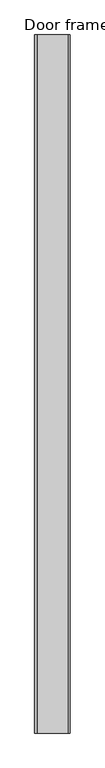
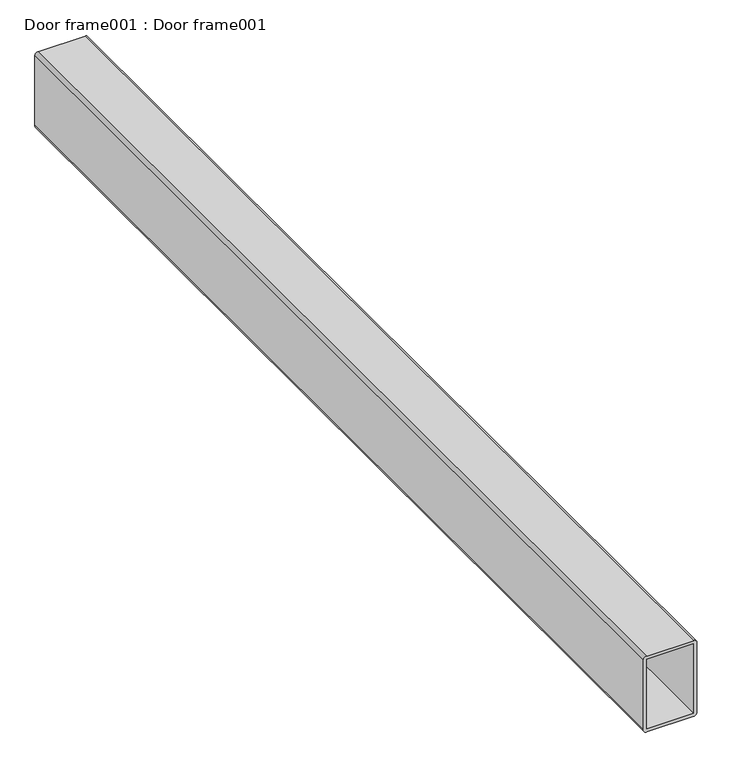
"""IFC4 building model written with IfcOpenShell, lengths in millimetres: proxy geometry, Door frame001 : Door frame001."""

import ifcopenshell
import ifcopenshell.guid

model = None  # the IFC model being written
_history = None  # IfcOwnerHistory: only IFC2X3 demands one
_inside = {}  # id of a spatial element -> (the spatial element, [elements in it])
_under = {}  # id of a project, library or spatial element -> (it, [spatial elements below it])
_declared = {}  # id of a project -> (the project, [libraries it declares])
_typed = {}  # id of a type object -> (the type object, [elements of that type])
_made_of = {}  # id of a material, layer set ... -> (it, [elements and type objects made of it])


def new_model(schema):
    """Start an empty IFC model of exactly this schema.

    Asked for "IFC4X3", IfcOpenShell would pick the latest addendum, in which some entities
    have other attributes; the version numbers below select the first issue.
    IFC2X3 requires an IfcOwnerHistory on every rooted entity: one is made here for all.
    """
    global model, _history
    if schema == "IFC4X3":
        model = ifcopenshell.file(schema_version=(4, 3, 0, 0))
    else:
        model = ifcopenshell.file(schema=schema)
    _inside.clear()
    _under.clear()
    _declared.clear()
    _typed.clear()
    _made_of.clear()
    _history = None
    if model.schema == "IFC2X3":
        org = make("IfcOrganization", Name="unknown")
        user = make(
            "IfcPersonAndOrganization",
            ThePerson=make("IfcPerson", FamilyName="unknown"),
            TheOrganization=org,
        )
        app = make(
            "IfcApplication",
            ApplicationDeveloper=org,
            Version="unknown",
            ApplicationFullName="unknown",
            ApplicationIdentifier="unknown",
        )
        _history = make(
            "IfcOwnerHistory",
            OwningUser=user,
            OwningApplication=app,
            ChangeAction="ADDED",
            CreationDate=0,
        )
    return model


def make(cls, **values):
    """One entity of the class cls with the attributes given. An attribute that is None is left unset."""
    return model.create_entity(
        cls, **{name: value for name, value in values.items() if value is not None}
    )


def rooted(cls, **values):
    """An entity with a GlobalId (a new one), such as an element, a storey or a relation."""
    return make(cls, GlobalId=ifcopenshell.guid.new(), OwnerHistory=_history, **values)


def si_unit(unit_type, name, prefix=None):
    """IfcSIUnit, for example si_unit("LENGTHUNIT", "METRE", prefix="MILLI")."""
    return make("IfcSIUnit", UnitType=unit_type, Prefix=prefix, Name=name)


def assignment(units):
    """IfcUnitAssignment: the units of a project."""
    return None if units is None else make("IfcUnitAssignment", Units=units)


def point(xyz):
    """IfcCartesianPoint."""
    return None if xyz is None else make("IfcCartesianPoint", Coordinates=xyz)


def direction(xyz):
    """IfcDirection."""
    return None if xyz is None else make("IfcDirection", DirectionRatios=xyz)


def frame(location, z_axis=None, x_axis=None):
    """IfcAxis2Placement3D, a coordinate frame: its origin and axes. An axis left out is left unset."""
    return make(
        "IfcAxis2Placement3D",
        Location=point(location),
        Axis=direction(z_axis),
        RefDirection=direction(x_axis),
    )


def frame_2d(location, x_axis=None):
    """IfcAxis2Placement2D, a coordinate frame in the plane: its origin and x axis."""
    return make(
        "IfcAxis2Placement2D", Location=point(location), RefDirection=direction(x_axis)
    )


def origin():
    """The frame at (0, 0, 0) with its axes left unset."""
    return frame((0.0, 0.0, 0.0))


def place(relative_to, where):
    """IfcLocalPlacement: puts the frame where relative to a parent placement (None: the world)."""
    return make(
        "IfcLocalPlacement", PlacementRelTo=relative_to, RelativePlacement=where
    )


def context(
    kind, dimensions, precision=None, world=None, true_north=None, identifier=None
):
    """IfcGeometricRepresentationContext, for example the 3D "Model" context."""
    return make(
        "IfcGeometricRepresentationContext",
        ContextIdentifier=identifier,
        ContextType=kind,
        CoordinateSpaceDimension=dimensions,
        Precision=precision,
        WorldCoordinateSystem=world,
        TrueNorth=true_north,
    )


def project(units=None, contexts=None):
    """IfcProject with its units and contexts."""
    return rooted(
        "IfcProject",
        Name="project",
        RepresentationContexts=contexts,
        UnitsInContext=assignment(units),
    )


def spatial(cls, under=None, at=None, **own):
    """A site, building, storey or space (cls), placed at a placement, below another one or the project."""
    s = rooted(cls, ObjectPlacement=at, **own)
    if under is not None:
        _under.setdefault(under.id(), (under, []))[1].append(s)
    return s


def polyline(points):
    """IfcPolyline through the points."""
    return make("IfcPolyline", Points=[point(p) for p in points])


def circle_curve(where, radius):
    """IfcCircle in the frame where."""
    return make("IfcCircle", Position=where, Radius=radius)


def trimmed(basis, trim1, trim2, sense, master):
    """IfcTrimmedCurve: the piece of a basis curve between two trims."""
    return make(
        "IfcTrimmedCurve",
        BasisCurve=basis,
        Trim1=trim1,
        Trim2=trim2,
        SenseAgreement=sense,
        MasterRepresentation=master,
    )


def segment(curve, same_sense, transition):
    """IfcCompositeCurveSegment."""
    return make(
        "IfcCompositeCurveSegment",
        Transition=transition,
        SameSense=same_sense,
        ParentCurve=curve,
    )


def composite_curve(segments, self_intersect=None):
    """IfcCompositeCurve: segments joined end to end."""
    return make("IfcCompositeCurve", Segments=segments, SelfIntersect=self_intersect)


def outline(outer, holes=None, kind="AREA"):
    """IfcArbitraryClosedProfileDef: a profile drawn as a closed curve; with holes, ...WithVoids."""
    if holes is None:
        return make("IfcArbitraryClosedProfileDef", ProfileType=kind, OuterCurve=outer)
    return make(
        "IfcArbitraryProfileDefWithVoids",
        ProfileType=kind,
        OuterCurve=outer,
        InnerCurves=holes,
    )


def extrude(swept, where, along, depth):
    """IfcExtrudedAreaSolid: the profile swept, set in the frame where, extruded along a direction by depth."""
    return make(
        "IfcExtrudedAreaSolid",
        SweptArea=swept,
        Position=where,
        ExtrudedDirection=direction(along),
        Depth=depth,
    )


def shape(context_of_items, identifier, shape_type, items):
    """IfcShapeRepresentation: the items that make up one representation, for example the "Body"."""
    return make(
        "IfcShapeRepresentation",
        ContextOfItems=context_of_items,
        RepresentationIdentifier=identifier,
        RepresentationType=shape_type,
        Items=items,
    )


def source(mapping_origin, context_of_items, identifier, shape_type, items):
    """IfcRepresentationMap: a shape defined once, which mapped items show again and again."""
    return make(
        "IfcRepresentationMap",
        MappingOrigin=mapping_origin,
        MappedRepresentation=shape(context_of_items, identifier, shape_type, items),
    )


def transform(
    local_origin,
    x_axis=None,
    y_axis=None,
    z_axis=None,
    scale=None,
    scale2=None,
    scale3=None,
    uniform=True,
):
    """IfcCartesianTransformationOperator3D, or its non-uniform kind. x_axis, y_axis, z_axis: its Axis1, 2, 3."""
    if uniform:
        return make(
            "IfcCartesianTransformationOperator3D",
            Axis1=direction(x_axis),
            Axis2=direction(y_axis),
            LocalOrigin=point(local_origin),
            Scale=scale,
            Axis3=direction(z_axis),
        )
    return make(
        "IfcCartesianTransformationOperator3DnonUniform",
        Axis1=direction(x_axis),
        Axis2=direction(y_axis),
        LocalOrigin=point(local_origin),
        Scale=scale,
        Axis3=direction(z_axis),
        Scale2=scale2,
        Scale3=scale3,
    )


def mapped(mapping_source, mapping_target):
    """IfcMappedItem: shows the shape of a source again, moved by a transform."""
    return make(
        "IfcMappedItem", MappingSource=mapping_source, MappingTarget=mapping_target
    )


def made_of(thing, what):
    """Note that an element or type object is made of a material, layer set ...; save() writes the relation."""
    if what is not None:
        _made_of.setdefault(what.id(), (what, []))[1].append(thing)
    return thing


def element(
    cls,
    number,
    at=None,
    inside=None,
    cuts=None,
    type_object=None,
    material=None,
    context=None,
    identifier="Body",
    shape_type=None,
    held_by="IfcProductDefinitionShape",
    body=None,
    shapes=None,
    **own,
):
    """One element of the class cls, such as IfcWall. Its Tag is "e" and its number.

    at: its placement. inside: the storey or other place that contains it. cuts: it is an
    opening in that element (IfcRelVoidsElement). A single representation is given by context,
    identifier, shape_type and body (its items); several are given by shapes. held_by: the class
    of the entity that holds the representations. save() writes the other relations.
    """
    e = rooted(cls, Tag="e%d" % number, ObjectPlacement=at, **own)
    if body is not None:
        shapes = [shape(context, identifier, shape_type, body)]
    if shapes is not None:
        e.Representation = make(held_by, Representations=shapes)
    if inside is not None:
        _inside.setdefault(inside.id(), (inside, []))[1].append(e)
    if cuts is not None:
        rooted(
            "IfcRelVoidsElement", RelatingBuildingElement=cuts, RelatedOpeningElement=e
        )
    if type_object is not None:
        _typed.setdefault(type_object.id(), (type_object, []))[1].append(e)
    return made_of(e, material)


def aggregate(whole, parts):
    """IfcRelAggregates: a whole, such as a stair, and the parts it consists of."""
    return rooted("IfcRelAggregates", RelatingObject=whole, RelatedObjects=parts)


def save(model, path):
    """Write the relations noted so far, then the file.

    IfcRelAggregates (storeys below a building ...), IfcRelContainedInSpatialStructure (elements
    in a storey), IfcRelDefinesByType, IfcRelAssociatesMaterial and IfcRelDeclares: one each for
    every whole, place, type object, material and project.
    """
    for whole, parts in _under.values():
        aggregate(whole, parts)
    for where, things in _inside.values():
        rooted(
            "IfcRelContainedInSpatialStructure",
            RelatedElements=things,
            RelatingStructure=where,
        )
    for kind, things in _typed.values():
        rooted("IfcRelDefinesByType", RelatedObjects=things, RelatingType=kind)
    for what, things in _made_of.values():
        rooted("IfcRelAssociatesMaterial", RelatedObjects=things, RelatingMaterial=what)
    for by, libraries in _declared.values():
        rooted("IfcRelDeclares", RelatingContext=by, RelatedDefinitions=libraries)
    model.write(path)


def door_frame001_door_frame001_2a17c90b(model_context):
    return source(origin(), model_context, "Body", "SweptSolid", [
        extrude(outline(composite_curve([segment(polyline([(32616.0375625, -8390.3106967), (32616.0375625, -8301.4106967)]), True, "CONTINUOUS"), segment(trimmed(circle_curve(frame_2d((32622.3875625, -8301.4106967)), 6.35), [point((32616.0375625, -8301.4106967))], [point((32622.3875625, -8295.0606967))], False, "CARTESIAN"), True, "CONTINUOUS"), segment(polyline([(32622.3875625, -8295.0606967), (32762.0875625, -8295.0606967)]), True, "CONTINUOUS"), segment(trimmed(circle_curve(frame_2d((32762.0875625, -8301.4106967)), 6.35), [point((32762.0875625, -8295.0606967))], [point((32768.4375625, -8301.4106967))], False, "CARTESIAN"), True, "CONTINUOUS"), segment(polyline([(32768.4375625, -8301.4106967), (32768.4375625, -8390.3106967)]), True, "CONTINUOUS"), segment(trimmed(circle_curve(frame_2d((32762.0875625, -8390.3106967)), 6.35), [point((32768.4375625, -8390.3106967))], [point((32762.0875625, -8396.6606967))], False, "CARTESIAN"), True, "CONTINUOUS"), segment(polyline([(32762.0875625, -8396.6606967), (32622.3875625, -8396.6606967)]), True, "CONTINUOUS"), segment(trimmed(circle_curve(frame_2d((32622.3875625, -8390.3106967)), 6.35), [point((32622.3875625, -8396.6606967))], [point((32616.0375625, -8390.3106967))], False, "CARTESIAN"), True, "CONTINUOUS")], self_intersect=False), holes=[polyline([(32761.9375625, -8301.5606967), (32622.5375625, -8301.5606967), (32622.5375625, -8390.1606967), (32761.9375625, -8390.1606967), (32761.9375625, -8301.5606967)])]), frame((0.0, 4540.4513244, 0.0), z_axis=(0.0, 1.0, 0.0), x_axis=(0.0, 0.0, 1.0)), (0.0, 0.0, 1.0), 2000.0),
    ])


if __name__ == "__main__":
    model = new_model("IFC4")
    model_context = context("Model", 3, world=origin())
    ifc_project = project(units=[si_unit("LENGTHUNIT", "METRE", prefix="MILLI")], contexts=[model_context])
    site = spatial("IfcSite", under=ifc_project)
    building = spatial("IfcBuilding", under=site)
    placement = place(None, origin())
    door_frame001_door_frame001_shape = door_frame001_door_frame001_2a17c90b(model_context)
    element("IfcBuildingElementProxy", 1, Name="Door frame001 : Door frame001", ObjectType="Door frame001 : Door frame001", at=placement, inside=building, context=model_context, shape_type="MappedRepresentation", body=[
        mapped(door_frame001_door_frame001_shape, transform((0.0, 0.0, 0.0), x_axis=(1.0, 0.0, 0.0), y_axis=(0.0, 1.0, 0.0), z_axis=(0.0, 0.0, 1.0))),
    ])
    save(model, "model.ifc")

# Revit data of these elements
# Type "Door frame001 : Door frame001"
#   NameOverride = "Door frame001"
# Element 1 (IfcBuildingElementProxy, "Door frame001 : Door frame001")
#   Materials on its faces: "DOOR FRAME: TUBE STEEL PROFILE - METALIZED, PRIMED & PAINTED (COLOR PER ARCHITECT)"
# Materials
#   "DOOR FRAME: TUBE STEEL PROFILE - METALIZED, PRIMED & PAINTED (COLOR PER ARCHITECT)": class "Unassigned", colour RGB 128 128 128, transparency 0, Cost = 0
